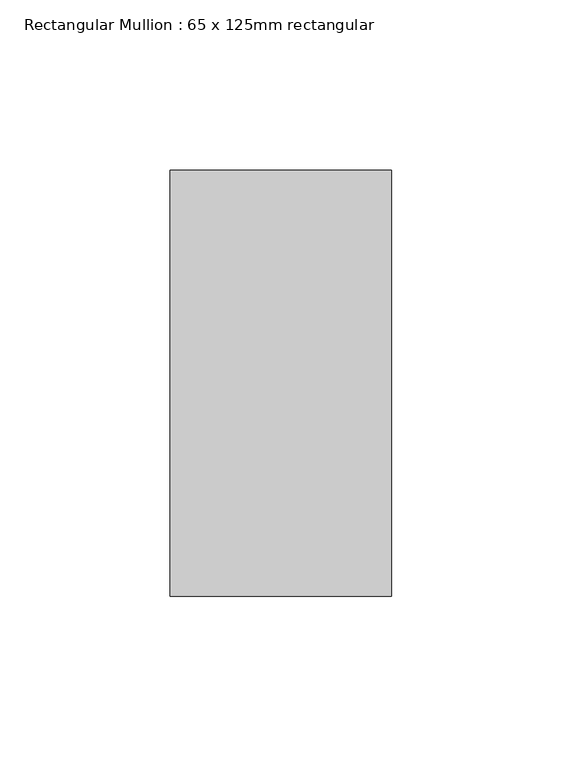
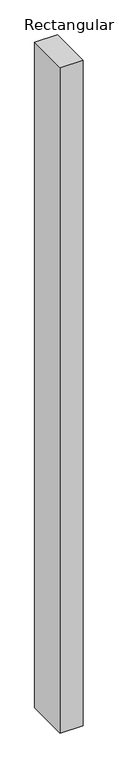
"""IFC4 building model written with IfcOpenShell, lengths in millimetres: member geometry, Rectangular Mullion : 65 x 125mm rectangular."""

from ifc_helpers import new_model, si_unit, frame, origin, place, context, project, spatial, polyline, outline, extrude, source, transform, mapped, element, save


def rectangular_mullion_65_x_125mm_rectangular_b62c991d(model_context):
    return source(origin(), model_context, "Body", "SweptSolid", [
        extrude(outline(polyline([(32.5, 62.5), (32.5, -62.5), (-32.5, -62.5), (-32.5, 62.5), (32.5, 62.5)])), frame((0.0, 0.0, -2000.0), z_axis=(0.0, 0.0, 1.0), x_axis=(1.0, 0.0, 0.0)), (0.0, 0.0, 1.0), 2000.0),
    ])


if __name__ == "__main__":
    model = new_model("IFC4")
    model_context = context("Model", 3, world=origin())
    ifc_project = project(units=[si_unit("LENGTHUNIT", "METRE", prefix="MILLI")], contexts=[model_context])
    site = spatial("IfcSite", under=ifc_project)
    building = spatial("IfcBuilding", under=site)
    placement = place(None, origin())
    rectangular_mullion_65_x_125mm_rectangular_shape = rectangular_mullion_65_x_125mm_rectangular_b62c991d(model_context)
    element("IfcMember", 1, ObjectType="Rectangular Mullion : 65 x 125mm rectangular", at=placement, inside=building, context=model_context, shape_type="MappedRepresentation", body=[
        mapped(rectangular_mullion_65_x_125mm_rectangular_shape, transform((0.0, 0.0, 0.0), x_axis=(1.0, 0.0, 0.0), y_axis=(0.0, 1.0, 0.0), z_axis=(0.0, 0.0, 1.0))),
    ])
    save(model, "model.ifc")

# Revit data of these elements
# Type "Rectangular Mullion : 65 x 125mm rectangular"
#   built-in parameter 1007304 = 0.410105 (stored number, unit not read)
#   built-in parameter 1007301 = 0.106627 (stored number, unit not read)
#   built-in parameter 1007300 = 0.106627 (stored number, unit not read)
# Element 1 (IfcMember, "Rectangular Mullion : 65 x 125mm rectangular")
#   Materials on its faces: "Aluminum"
# Materials
#   "Aluminum": class "Metal", colour RGB 244 245 246, transparency 0, Description = "Aluminum 6061", Cost = 0
